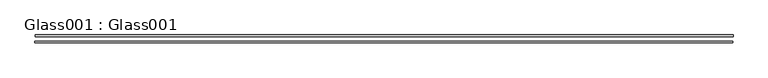
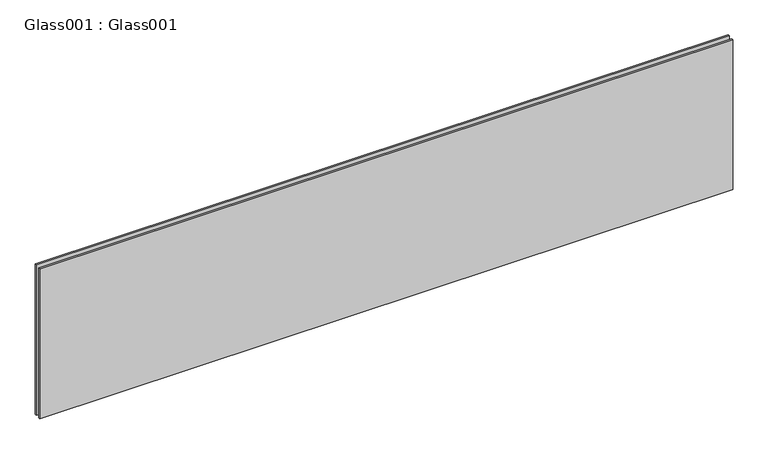
"""IFC4 building model written with IfcOpenShell, lengths in millimetres: proxy geometry, Glass001 : Glass001."""

from ifc_helpers import new_model, si_unit, frame, origin, place, context, project, spatial, polyline, outline, extrude, source, transform, mapped, element, save


def glass001_glass001_dcca6a89(model_context):
    return source(origin(), model_context, "Body", "SweptSolid", [
        extrude(outline(polyline([(14384.0178845, -4642.8027938), (14384.0178845, -4647.8027938), (12384.0178845, -4647.8027938), (12384.0178845, -4642.8027938), (14384.0178845, -4642.8027938)])), frame((0.0, 0.0, 38486.2565625), z_axis=(0.0, 0.0, 1.0), x_axis=(1.0, 0.0, 0.0)), (0.0, 0.0, 1.0), 457.9389687),
        extrude(outline(polyline([(14383.0178845, -4660.8027938), (14383.0178845, -4665.8027938), (12383.0178845, -4665.8027938), (12383.0178845, -4660.8027938), (14383.0178845, -4660.8027938)])), frame((0.0, 0.0, 38486.2565625), z_axis=(0.0, 0.0, 1.0), x_axis=(1.0, 0.0, 0.0)), (0.0, 0.0, 1.0), 457.9389687),
    ])


if __name__ == "__main__":
    model = new_model("IFC4")
    model_context = context("Model", 3, world=origin())
    ifc_project = project(units=[si_unit("LENGTHUNIT", "METRE", prefix="MILLI")], contexts=[model_context])
    site = spatial("IfcSite", under=ifc_project)
    building = spatial("IfcBuilding", under=site)
    placement = place(None, origin())
    glass001_glass001_shape = glass001_glass001_dcca6a89(model_context)
    element("IfcBuildingElementProxy", 1, Name="Glass001 : Glass001", ObjectType="Glass001 : Glass001", at=placement, inside=building, context=model_context, shape_type="MappedRepresentation", body=[
        mapped(glass001_glass001_shape, transform((0.0, 0.0, 0.0), x_axis=(1.0, 0.0, 0.0), y_axis=(0.0, 1.0, 0.0), z_axis=(0.0, 0.0, 1.0))),
    ])
    save(model, "model.ifc")

# Revit data of these elements
# Type "Glass001 : Glass001"
#   NameOverride = "Glass001"
# Element 1 (IfcBuildingElementProxy, "Glass001 : Glass001")
#   Materials on its faces: "1\" INSULATED GLAZING"
# Materials
#   "1\" INSULATED GLAZING": class "Unassigned", colour RGB 146 199 212, transparency 0
